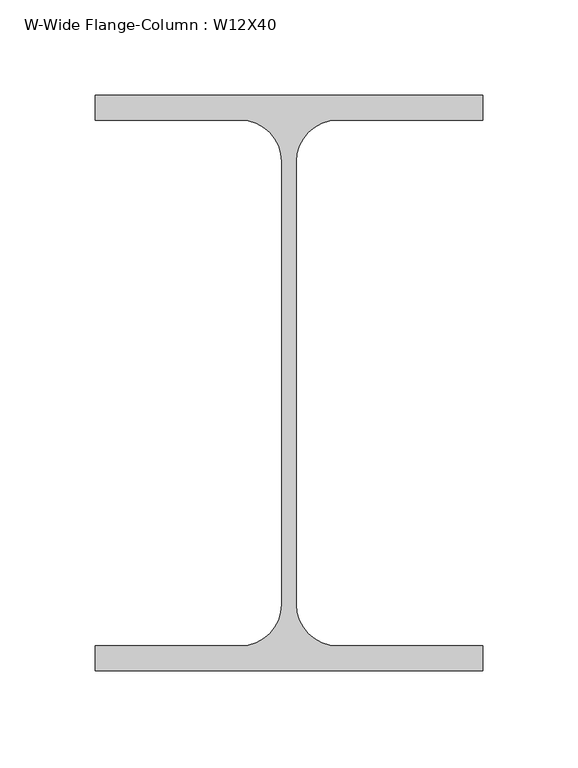
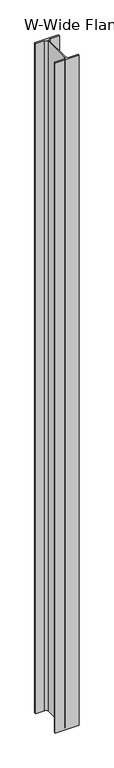
"""IFC4 building model written with IfcOpenShell, lengths in millimetres: column geometry, W-Wide Flange-Column : W12X40."""

from ifc_helpers import new_model, si_unit, point, frame, frame_2d, origin, place, context, project, spatial, polyline, circle_curve, trimmed, segment, composite_curve, outline, extrude, source, transform, mapped, element, save


def w_wide_flange_column_w12x40_e5d2a7b0(model_context):
    return source(origin(), model_context, "Body", "SweptSolid", [
        extrude(outline(composite_curve([segment(polyline([(101.727, 151.13), (101.727, 138.049), (25.5905, 138.049)]), True, "CONTINUOUS"), segment(trimmed(circle_curve(frame_2d((25.5905, 116.205)), 21.844), [point((25.5905, 138.049))], [point((3.7465, 116.205))], True, "CARTESIAN"), True, "CONTINUOUS"), segment(polyline([(3.7465, 116.205), (3.7465, -116.205)]), True, "CONTINUOUS"), segment(trimmed(circle_curve(frame_2d((25.5905, -116.205)), 21.844), [point((3.7465, -116.205))], [point((25.5905, -138.049))], True, "CARTESIAN"), True, "CONTINUOUS"), segment(polyline([(25.5905, -138.049), (101.727, -138.049), (101.727, -151.13), (-101.727, -151.13), (-101.727, -138.049), (-25.5905, -138.049)]), True, "CONTINUOUS"), segment(trimmed(circle_curve(frame_2d((-25.5905, -116.205)), 21.844), [point((-25.5905, -138.049))], [point((-3.7465, -116.205))], True, "CARTESIAN"), True, "CONTINUOUS"), segment(polyline([(-3.7465, -116.205), (-3.7465, 116.205)]), True, "CONTINUOUS"), segment(trimmed(circle_curve(frame_2d((-25.5905, 116.205)), 21.844), [point((-3.7465, 116.205))], [point((-25.5905, 138.049))], True, "CARTESIAN"), True, "CONTINUOUS"), segment(polyline([(-25.5905, 138.049), (-101.727, 138.049), (-101.727, 151.13), (101.727, 151.13)]), True, "CONTINUOUS")], self_intersect=False)), frame((0.0, 0.0, 23317.2), z_axis=(0.0, 0.0, 1.0), x_axis=(1.0, 0.0, 0.0)), (0.0, 0.0, 1.0), 6013.45),
    ])


if __name__ == "__main__":
    model = new_model("IFC4")
    model_context = context("Model", 3, world=origin())
    ifc_project = project(units=[si_unit("LENGTHUNIT", "METRE", prefix="MILLI")], contexts=[model_context])
    site = spatial("IfcSite", under=ifc_project)
    building = spatial("IfcBuilding", under=site)
    placement = place(None, origin())
    w_wide_flange_column_w12x40_shape = w_wide_flange_column_w12x40_e5d2a7b0(model_context)
    element("IfcColumn", 1, ObjectType="W-Wide Flange-Column : W12X40", at=placement, inside=building, context=model_context, shape_type="MappedRepresentation", body=[
        mapped(w_wide_flange_column_w12x40_shape, transform((0.0, 0.0, 0.0), x_axis=(1.0, 0.0, 0.0), y_axis=(0.0, 1.0, 0.0), z_axis=(0.0, 0.0, 1.0))),
    ])
    save(model, "model.ifc")

# Revit data of these elements
# Type "W-Wide Flange-Column : W12X40"
#   Assembly Code = "B10"
#   W = 40
#   bf = 0' - 8.01"
#   d = 0' - 11.9"
#   k = 0' - 1 3/8"
#   kr = 0' - 0.86"
#   tf = 0' - 0.515"
#   tw = 0' - 0.295"
#   A = 0.08125 SF
#   Structural Material [instance default] = Steel ASTM A992
# Element 1 (IfcColumn, "W-Wide Flange-Column : W12X40")
#   Materials on its faces: "Steel ASTM A992"
# Materials
#   "Steel ASTM A992": class "Metal", colour RGB 199 199 199, transparency 0, Description = "Structural steel 50ksi", Cost = 0
